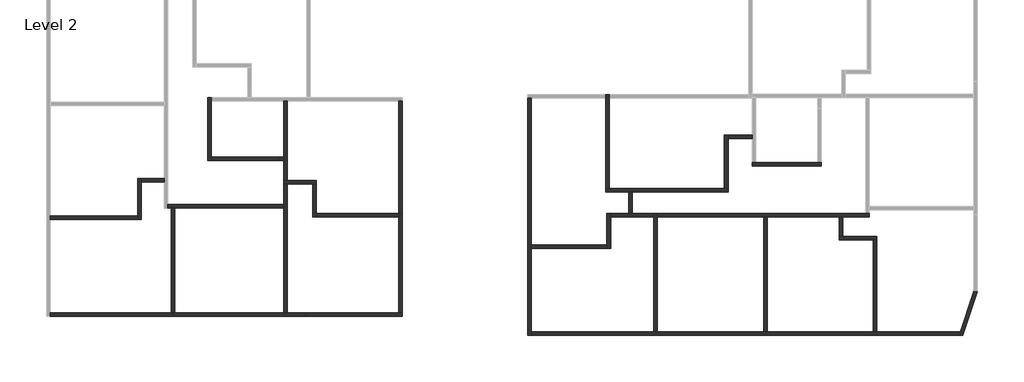
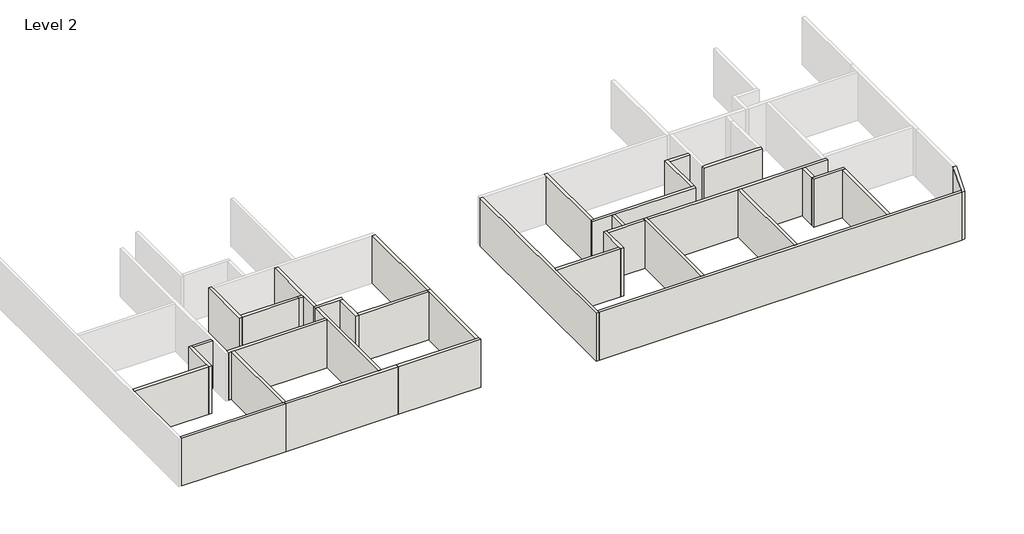
# One storey, part 1 of 2: 36 walls.
"""IFC4 building model written with IfcOpenShell, lengths in millimetres."""

from ifc_helpers import new_model, si_unit, frame, origin, place, context, project, spatial, polyline, outline, extrude, faceted_brep, element, save

model = new_model("IFC4")

# Units and contexts
model_context = context("Model", 3, world=origin())
ifc_project = project(units=[si_unit("LENGTHUNIT", "METRE", prefix="MILLI")], contexts=[model_context])

# Site, building, storey
site = spatial("IfcSite", under=ifc_project)
building = spatial("IfcBuilding", under=site)
storey = spatial("IfcBuildingStorey", under=building, Name="Level 2", Elevation=3000.0)

# Walls
placement = place(None, origin())
element("IfcWall", 1, ObjectType="Generic - 200mm", at=placement, inside=storey, context=model_context, shape_type="Brep", body=[
    faceted_brep([(21449.836337, -2276.2808257, 3000.0), (21249.836337, -2276.2808257, 3000.0), (17730.6041014, -2276.2808257, 3000.0), (17530.6041014, -2276.2808257, 3000.0), (17530.6041014, -2276.2808257, 6360.0), (17730.6041014, -2276.2808257, 6360.0), (21249.836337, -2276.2808257, 6360.0), (21449.836337, -2276.2808257, 6360.0), (21449.836337, -2476.2808257, 3000.0), (21449.836337, -2476.2808257, 6360.0), (17530.6041014, -2476.2808257, 6360.0), (17530.6041014, -2476.2808257, 3000.0)], [[[0, 1, 2, 3, 4, 5, 6, 7]], [[8, 9, 10, 11]], [[3, 2, 1, 0, 8, 11]], [[7, 6, 5, 4, 10, 9]], [[0, 7, 9, 8]], [[4, 3, 11, 10]]]),
])
element("IfcWall", 2, ObjectType="Generic - 200mm", at=placement, inside=storey, context=model_context, shape_type="SweptSolid", body=[
    extrude(outline(polyline([(18379.836337, -5340.0098119), (18379.836337, -11836.6907835), (18179.836337, -11836.6907835), (18179.836337, -5340.0098119), (18379.836337, -5340.0098119)])), frame((0.0, 0.0, 3000.0), z_axis=(0.0, 0.0, 1.0), x_axis=(1.0, 0.0, 0.0)), (0.0, 0.0, 1.0), 3360.0),
])
element("IfcWall", 3, ObjectType="Generic - 200mm", at=placement, inside=storey, context=model_context, shape_type="Brep", body=[
    faceted_brep([(29295.3124022, -11836.6907835, 3000.0), (24588.8612349, -11836.6907835, 3000.0), (24388.8612349, -11836.6907835, 3000.0), (18379.836337, -11836.6907835, 3000.0), (18179.836337, -11836.6907835, 3000.0), (12179.836337, -11836.6907835, 3000.0), (11979.836337, -11836.6907835, 3000.0), (5043.716007, -11836.6907835, 3000.0), (5043.716007, -11836.6907835, 6360.0), (11979.836337, -11836.6907835, 6360.0), (12179.836337, -11836.6907835, 6360.0), (18179.836337, -11836.6907835, 6360.0), (18379.836337, -11836.6907835, 6360.0), (24388.8612349, -11836.6907835, 6360.0), (24588.8612349, -11836.6907835, 6360.0), (29295.3124022, -11836.6907835, 6360.0), (29227.8162902, -12036.6907835, 3000.0), (29227.8162902, -12036.6907835, 6360.0), (5043.716007, -12036.6907835, 6360.0), (5043.716007, -12036.6907835, 3000.0)], [[[0, 1, 2, 3, 4, 5, 6, 7, 8, 9, 10, 11, 12, 13, 14, 15]], [[16, 17, 18, 19]], [[7, 6, 5, 4, 3, 2, 1, 0, 16, 19]], [[15, 14, 13, 12, 11, 10, 9, 8, 18, 17]], [[0, 15, 17, 16]], [[8, 7, 19, 18]]]),
])
element("IfcWall", 4, ObjectType="Generic - 200mm", at=placement, inside=storey, context=model_context, shape_type="Brep", body=[
    faceted_brep([(30069.3799498, -9543.0251929, 3000.0), (29295.3124022, -11836.6907835, 3000.0), (29227.8162902, -12036.6907835, 3000.0), (29227.8162902, -12036.6907835, 6360.0), (29295.3124022, -11836.6907835, 6360.0), (30069.3799498, -9543.0251929, 6360.0), (30269.3799498, -9575.863443, 3000.0), (30269.3799498, -9575.863443, 6360.0), (29438.8985612, -12036.6907835, 6360.0), (29438.8985612, -12036.6907835, 3000.0)], [[[0, 1, 2, 3, 4, 5]], [[6, 7, 8, 9]], [[2, 1, 0, 6, 9]], [[5, 4, 3, 8, 7]], [[0, 5, 7, 6]], [[3, 2, 9, 8]]]),
])
element("IfcWall", 5, ObjectType="Generic - 200mm", at=placement, inside=storey, context=model_context, shape_type="Brep", body=[
    faceted_brep([(24163.3998354, -5140.0098119, 3000.0), (24148.8612349, -5140.0098119, 3000.0), (23948.8612349, -5140.0098119, 3000.0), (12179.836337, -5140.0098119, 3000.0), (12179.836337, -5140.0098119, 6360.0), (23948.8612349, -5140.0098119, 6360.0), (24148.8612349, -5140.0098119, 6360.0), (24163.3998354, -5140.0098119, 6360.0), (24163.3998354, -5340.0098119, 3000.0), (24163.3998354, -5340.0098119, 6360.0), (22668.8612349, -5340.0098119, 6360.0), (22468.8612349, -5340.0098119, 6360.0), (18379.836337, -5340.0098119, 6360.0), (18179.836337, -5340.0098119, 6360.0), (12179.836337, -5340.0098119, 6360.0), (12179.836337, -5340.0098119, 3000.0), (18179.836337, -5340.0098119, 3000.0), (18379.836337, -5340.0098119, 3000.0), (22468.8612349, -5340.0098119, 3000.0), (22668.8612349, -5340.0098119, 3000.0)], [[[0, 1, 2, 3, 4, 5, 6, 7]], [[8, 9, 10, 11, 12, 13, 14, 15, 16, 17, 18, 19]], [[3, 2, 1, 0, 8, 19, 18, 17, 16, 15]], [[7, 6, 5, 4, 14, 13, 12, 11, 10, 9]], [[0, 7, 9, 8]], [[4, 3, 15, 14]]]),
])
element("IfcWall", 6, ObjectType="Generic - 200mm", at=placement, inside=storey, context=model_context, shape_type="Brep", body=[
    faceted_brep([(4843.716007, 1379.9901881, 3000.0), (4843.716007, -12036.6907835, 3000.0), (4843.716007, -12036.6907835, 6360.0), (4843.716007, 1379.9901881, 6360.0), (5043.716007, 1379.9901881, 3000.0), (5043.716007, 1379.9901881, 6360.0), (5043.716007, -6920.0098119, 6360.0), (5043.716007, -7120.0098119, 6360.0), (5043.716007, -11836.6907835, 6360.0), (5043.716007, -12036.6907835, 6360.0), (5043.716007, -12036.6907835, 3000.0), (5043.716007, -11836.6907835, 3000.0), (5043.716007, -7120.0098119, 3000.0), (5043.716007, -6920.0098119, 3000.0)], [[[0, 1, 2, 3]], [[4, 5, 6, 7, 8, 9, 10, 11, 12, 13]], [[1, 0, 4, 13, 12, 11, 10]], [[3, 2, 9, 8, 7, 6, 5]], [[2, 1, 10, 9]], [[0, 3, 5, 4]]]),
])
element("IfcWall", 7, ObjectType="Generic - 200mm", at=placement, inside=storey, context=model_context, shape_type="Brep", body=[
    faceted_brep([(9268.8612349, -3940.0098119, 3000.0), (10568.8612349, -3940.0098119, 3000.0), (10768.8612349, -3940.0098119, 3000.0), (16170.6041014, -3940.0098119, 3000.0), (16170.6041014, -3940.0098119, 6360.0), (10768.8612349, -3940.0098119, 6360.0), (10568.8612349, -3940.0098119, 6360.0), (9268.8612349, -3940.0098119, 6360.0), (9268.8612349, -3740.0098119, 3000.0), (9268.8612349, -3740.0098119, 6360.0), (9468.8612349, -3740.0098119, 6360.0), (15970.6041014, -3740.0098119, 6360.0), (16170.6041014, -3740.0098119, 6360.0), (16170.6041014, -3740.0098119, 3000.0), (15970.6041014, -3740.0098119, 3000.0), (9468.8612349, -3740.0098119, 3000.0), (16170.6041014, -3894.2728831, 3000.0)], [[[0, 1, 2, 3, 4, 5, 6, 7]], [[8, 9, 10, 11, 12, 13, 14, 15]], [[3, 2, 1, 0, 8, 15, 14, 13, 16]], [[7, 6, 5, 4, 12, 11, 10, 9]], [[4, 3, 16, 13, 12]], [[0, 7, 9, 8]]]),
])
element("IfcWall", 8, ObjectType="Generic - 200mm", at=placement, inside=storey, context=model_context, shape_type="Brep", body=[
    faceted_brep([(16170.6041014, -3740.0098119, 3000.0), (16170.6041014, -3694.2728831, 3000.0), (16170.6041014, -920.524372, 3000.0), (16170.6041014, -720.524372, 3000.0), (16170.6041014, -720.524372, 6360.0), (16170.6041014, -920.524372, 6360.0), (16170.6041014, -3740.0098119, 6360.0), (15970.6041014, -3740.0098119, 3000.0), (15970.6041014, -3740.0098119, 6360.0), (15970.6041014, -720.524372, 6360.0), (15970.6041014, -720.524372, 3000.0)], [[[0, 1, 2, 3, 4, 5, 6]], [[7, 8, 9, 10]], [[3, 2, 1, 0, 7, 10]], [[6, 5, 4, 9, 8]], [[0, 6, 8, 7]], [[4, 3, 10, 9]]]),
])
element("IfcWall", 9, ObjectType="Generic - 200mm", at=placement, inside=storey, context=model_context, shape_type="SweptSolid", body=[
    extrude(outline(polyline([(17530.6041014, -920.524372), (16170.6041014, -920.524372), (16170.6041014, -720.524372), (17530.6041014, -720.524372), (17530.6041014, -920.524372)])), frame((0.0, 0.0, 3000.0), z_axis=(0.0, 0.0, 1.0), x_axis=(1.0, 0.0, 0.0)), (0.0, 0.0, 1.0), 3360.0),
])
element("IfcWall", 10, ObjectType="Generic - 200mm", at=placement, inside=storey, context=model_context, shape_type="Brep", body=[
    faceted_brep([(22468.8612349, -6641.2808257, 3000.0), (24388.8612349, -6641.2808257, 3000.0), (24588.8612349, -6641.2808257, 3000.0), (24588.8612349, -6641.2808257, 6360.0), (24388.8612349, -6641.2808257, 6360.0), (22468.8612349, -6641.2808257, 6360.0), (22468.8612349, -6441.2808257, 3000.0), (22468.8612349, -6441.2808257, 6360.0), (22668.8612349, -6441.2808257, 6360.0), (24588.8612349, -6441.2808257, 6360.0), (24588.8612349, -6441.2808257, 3000.0), (22668.8612349, -6441.2808257, 3000.0)], [[[0, 1, 2, 3, 4, 5]], [[6, 7, 8, 9, 10, 11]], [[2, 1, 0, 6, 11, 10]], [[5, 4, 3, 9, 8, 7]], [[3, 2, 10, 9]], [[0, 5, 7, 6]]]),
])
element("IfcWall", 11, ObjectType="Generic - 200mm", at=placement, inside=storey, context=model_context, shape_type="SweptSolid", body=[
    extrude(outline(polyline([(24388.8612349, -11836.6907835), (24388.8612349, -6641.2808257), (24588.8612349, -6641.2808257), (24588.8612349, -11836.6907835), (24388.8612349, -11836.6907835)])), frame((0.0, 0.0, 3000.0), z_axis=(0.0, 0.0, 1.0), x_axis=(1.0, 0.0, 0.0)), (0.0, 0.0, 1.0), 3360.0),
])
element("IfcWall", 12, ObjectType="Generic - 200mm", at=placement, inside=storey, context=model_context, shape_type="SweptSolid", body=[
    extrude(outline(polyline([(22668.8612349, -5340.0098119), (22668.8612349, -6441.2808257), (22468.8612349, -6441.2808257), (22468.8612349, -5340.0098119), (22668.8612349, -5340.0098119)])), frame((0.0, 0.0, 3000.0), z_axis=(0.0, 0.0, 1.0), x_axis=(1.0, 0.0, 0.0)), (0.0, 0.0, 1.0), 3360.0),
])
element("IfcWall", 13, ObjectType="Generic - 200mm", at=placement, inside=storey, context=model_context, shape_type="Brep", body=[
    faceted_brep([(9268.8612349, 1579.9901881, 3000.0), (9268.8612349, 1379.9901881, 3000.0), (9268.8612349, -3740.0098119, 3000.0), (9268.8612349, -3740.0098119, 6360.0), (9268.8612349, 1379.9901881, 6360.0), (9268.8612349, 1579.9901881, 6360.0), (9468.8612349, 1579.9901881, 3000.0), (9468.8612349, 1579.9901881, 6360.0), (9468.8612349, 1579.475628, 6360.0), (9468.8612349, 1379.475628, 6360.0), (9468.8612349, -3740.0098119, 6360.0), (9468.8612349, -3740.0098119, 3000.0), (9468.8612349, 1379.475628, 3000.0), (9468.8612349, 1579.475628, 3000.0)], [[[0, 1, 2, 3, 4, 5]], [[6, 7, 8, 9, 10, 11, 12, 13]], [[2, 1, 0, 6, 13, 12, 11]], [[5, 4, 3, 10, 9, 8, 7]], [[3, 2, 11, 10]], [[0, 5, 7, 6]]]),
])
element("IfcWall", 14, ObjectType="Generic - 200mm", at=placement, inside=storey, context=model_context, shape_type="SweptSolid", body=[
    extrude(outline(polyline([(5043.716007, -6920.0098119), (9328.8612349, -6920.0098119), (9328.8612349, -7120.0098119), (5043.716007, -7120.0098119), (5043.716007, -6920.0098119)])), frame((0.0, 0.0, 3000.0), z_axis=(0.0, 0.0, 1.0), x_axis=(1.0, 0.0, 0.0)), (0.0, 0.0, 1.0), 3360.0),
])
element("IfcWall", 15, ObjectType="Generic - 200mm", at=placement, inside=storey, context=model_context, shape_type="Brep", body=[
    faceted_brep([(-2430.3449834, -5140.1378151, 3000.0), (-2430.3449834, -5340.1378151, 3000.0), (-2430.3449834, -10758.643998, 3000.0), (-2430.3449834, -10758.643998, 6360.0), (-2430.3449834, -5340.1378151, 6360.0), (-2430.3449834, -5140.1378151, 6360.0), (-2230.3449834, -5140.1378151, 3000.0), (-2230.3449834, -5140.1378151, 6360.0), (-2230.3449834, -10758.643998, 6360.0), (-2230.3449834, -10758.643998, 3000.0)], [[[0, 1, 2, 3, 4, 5]], [[6, 7, 8, 9]], [[2, 1, 0, 6, 9]], [[5, 4, 3, 8, 7]], [[3, 2, 9, 8]], [[0, 5, 7, 6]]]),
])
element("IfcWall", 16, ObjectType="Generic - 200mm", at=placement, inside=storey, context=model_context, shape_type="Brep", body=[
    faceted_brep([(-2230.3449834, -10758.643998, 3000.0), (-2430.3449834, -10758.643998, 3000.0), (-7730.3449834, -10758.643998, 3000.0), (-7730.3449834, -10758.643998, 6360.0), (-2430.3449834, -10758.643998, 6360.0), (-2230.3449834, -10758.643998, 6360.0), (-2230.3449834, -10958.643998, 3000.0), (-2230.3449834, -10958.643998, 6360.0), (-7730.3449834, -10958.643998, 6360.0), (-7730.3449834, -10958.643998, 3000.0), (-7730.3449834, -10932.392509, 3000.0), (-7730.3449834, -10759.1627129, 3000.0), (-7730.3449834, -10759.1627129, 6360.0)], [[[0, 1, 2, 3, 4, 5]], [[6, 7, 8, 9]], [[2, 1, 0, 6, 9, 10, 11]], [[3, 2, 11, 10, 9, 8, 12]], [[5, 4, 3, 12, 8, 7]], [[0, 5, 7, 6]]]),
])
element("IfcWall", 17, ObjectType="Generic - 200mm", at=placement, inside=storey, context=model_context, shape_type="Brep", body=[
    faceted_brep([(-7730.3449834, -10759.1627129, 3000.0), (-8730.3449834, -10759.1627129, 3000.0), (-8930.3449834, -10759.1627129, 3000.0), (-15109.8304233, -10759.1627129, 3000.0), (-15209.8304233, -10759.1627129, 3000.0), (-15209.8304233, -10759.1627129, 6360.0), (-15109.8304233, -10759.1627129, 6360.0), (-8930.3449834, -10759.1627129, 6360.0), (-8730.3449834, -10759.1627129, 6360.0), (-7730.3449834, -10759.1627129, 6360.0), (-7730.3449834, -10959.1627129, 3000.0), (-7730.3449834, -10959.1627129, 6360.0), (-15209.8304233, -10959.1627129, 6360.0), (-15209.8304233, -10959.1627129, 3000.0), (-7730.3449834, -10932.911224, 3000.0), (-7730.3449834, -10958.643998, 3000.0), (-15209.8304233, -10932.911224, 3000.0), (-15209.8304233, -10759.6814279, 3000.0), (-15209.8304233, -10759.6814279, 6360.0), (-7730.3449834, -10958.643998, 6360.0)], [[[0, 1, 2, 3, 4, 5, 6, 7, 8, 9]], [[10, 11, 12, 13]], [[4, 3, 2, 1, 0, 14, 15, 10, 13, 16, 17]], [[5, 4, 17, 16, 13, 12, 18]], [[9, 8, 7, 6, 5, 18, 12, 11, 19]], [[0, 9, 19, 11, 10, 15, 14]]]),
])
element("IfcWall", 18, ObjectType="Generic - 200mm", at=placement, inside=storey, context=model_context, shape_type="Brep", body=[
    faceted_brep([(-15209.8304233, -10759.6814279, 3000.0), (-15309.8304233, -10759.6814279, 3000.0), (-22146.5113948, -10759.6814279, 3000.0), (-22146.5113948, -10759.6814279, 6360.0), (-15309.8304233, -10759.6814279, 6360.0), (-15209.8304233, -10759.6814279, 6360.0), (-15209.8304233, -10959.6814279, 3000.0), (-15209.8304233, -10959.6814279, 6360.0), (-22146.5113948, -10959.6814279, 6360.0), (-22146.5113948, -10959.6814279, 3000.0), (-15209.8304233, -10933.429939, 3000.0), (-15209.8304233, -10959.1627129, 3000.0), (-15209.8304233, -10959.1627129, 6360.0)], [[[0, 1, 2, 3, 4, 5]], [[6, 7, 8, 9]], [[2, 1, 0, 10, 11, 6, 9]], [[5, 4, 3, 8, 7, 12]], [[0, 5, 12, 7, 6, 11, 10]], [[3, 2, 9, 8]]]),
])
element("IfcWall", 19, ObjectType="Generic - 200mm", at=placement, inside=storey, context=model_context, shape_type="Brep", body=[
    faceted_brep([(-13026.101437, -2140.1378151, 3000.0), (-13026.101437, -1940.1378151, 3000.0), (-13026.101437, 1200.8372871, 3000.0), (-13026.101437, 1400.8372871, 3000.0), (-13026.101437, 1400.8372871, 6360.0), (-13026.101437, 1200.8372871, 6360.0), (-13026.101437, -1940.1378151, 6360.0), (-13026.101437, -2140.1378151, 6360.0), (-13226.101437, -2140.1378151, 3000.0), (-13226.101437, -2140.1378151, 6360.0), (-13226.101437, 1400.8372871, 6360.0), (-13226.101437, 1400.8372871, 3000.0)], [[[0, 1, 2, 3, 4, 5, 6, 7]], [[8, 9, 10, 11]], [[3, 2, 1, 0, 8, 11]], [[7, 6, 5, 4, 10, 9]], [[0, 7, 9, 8]], [[4, 3, 11, 10]]]),
])
element("IfcWall", 20, ObjectType="Generic - 200mm", at=placement, inside=storey, context=model_context, shape_type="Brep", body=[
    faceted_brep([(-15489.8304233, -4839.1627129, 3000.0), (-15309.8304233, -4839.1627129, 3000.0), (-15109.8304233, -4839.1627129, 3000.0), (-8930.3449834, -4839.1627129, 3000.0), (-8930.3449834, -4839.1627129, 6360.0), (-15109.8304233, -4839.1627129, 6360.0), (-15309.8304233, -4839.1627129, 6360.0), (-15489.8304233, -4839.1627129, 6360.0), (-15489.8304233, -4639.1627129, 3000.0), (-15489.8304233, -4639.1627129, 6360.0), (-8930.3449834, -4639.1627129, 6360.0), (-8930.3449834, -4639.1627129, 3000.0)], [[[0, 1, 2, 3, 4, 5, 6, 7]], [[8, 9, 10, 11]], [[3, 2, 1, 0, 8, 11]], [[7, 6, 5, 4, 10, 9]], [[4, 3, 11, 10]], [[0, 7, 9, 8]]]),
])
element("IfcWall", 21, ObjectType="Generic - 200mm", at=placement, inside=storey, context=model_context, shape_type="SweptSolid", body=[
    extrude(outline(polyline([(-13026.101437, -1940.1378151), (-9250.3449834, -1940.1378151), (-9250.3449834, -2140.1378151), (-13026.101437, -2140.1378151), (-13026.101437, -1940.1378151)])), frame((0.0, 0.0, 3000.0), z_axis=(0.0, 0.0, 1.0), x_axis=(1.0, 0.0, 0.0)), (0.0, 0.0, 1.0), 3360.0),
])
element("IfcWall", 22, ObjectType="Generic - 200mm", at=placement, inside=storey, context=model_context, shape_type="SweptSolid", body=[
    extrude(outline(polyline([(-8930.3449834, -2140.1378151), (-9250.3449834, -2140.1378151), (-9250.3449834, -1940.1378151), (-8930.3449834, -1940.1378151), (-8930.3449834, -2140.1378151)])), frame((0.0, 0.0, 3000.0), z_axis=(0.0, 0.0, 1.0), x_axis=(1.0, 0.0, 0.0)), (0.0, 0.0, 1.0), 3360.0),
])
element("IfcWall", 23, ObjectType="Generic - 200mm", at=placement, inside=storey, context=model_context, shape_type="SweptSolid", body=[
    extrude(outline(polyline([(-2430.3449834, -5140.1378151), (-2430.3449834, 1200.8372871), (-2230.3449834, 1200.8372871), (-2230.3449834, -5140.1378151), (-2430.3449834, -5140.1378151)])), frame((0.0, 0.0, 3000.0), z_axis=(0.0, 0.0, 1.0), x_axis=(1.0, 0.0, 0.0)), (0.0, 0.0, 1.0), 3360.0),
])
element("IfcWall", 24, ObjectType="Generic - 200mm", at=placement, inside=storey, context=model_context, shape_type="Brep", body=[
    faceted_brep([(-8930.3449834, -3480.1378151, 3000.0), (-8730.3449834, -3480.1378151, 3000.0), (-7295.3449834, -3480.1378151, 3000.0), (-7095.3449834, -3480.1378151, 3000.0), (-7095.3449834, -3480.1378151, 6360.0), (-7295.3449834, -3480.1378151, 6360.0), (-8730.3449834, -3480.1378151, 6360.0), (-8930.3449834, -3480.1378151, 6360.0), (-8930.3449834, -3280.1378151, 3000.0), (-8930.3449834, -3280.1378151, 6360.0), (-8730.3449834, -3280.1378151, 6360.0), (-7095.3449834, -3280.1378151, 6360.0), (-7095.3449834, -3280.1378151, 3000.0), (-8730.3449834, -3280.1378151, 3000.0), (-8930.3449834, -3453.8863261, 3000.0)], [[[0, 1, 2, 3, 4, 5, 6, 7]], [[8, 9, 10, 11, 12, 13]], [[3, 2, 1, 0, 14, 8, 13, 12]], [[7, 6, 5, 4, 11, 10, 9]], [[0, 7, 9, 8, 14]], [[4, 3, 12, 11]]]),
])
element("IfcWall", 25, ObjectType="Generic - 200mm", at=placement, inside=storey, context=model_context, shape_type="Brep", body=[
    faceted_brep([(-8930.3449834, -3480.1378151, 3000.0), (-8930.3449834, -4639.1627129, 3000.0), (-8930.3449834, -4839.1627129, 3000.0), (-8930.3449834, -10759.1627129, 3000.0), (-8930.3449834, -10759.1627129, 6360.0), (-8930.3449834, -4839.1627129, 6360.0), (-8930.3449834, -4639.1627129, 6360.0), (-8930.3449834, -3480.1378151, 6360.0), (-8730.3449834, -3480.1378151, 3000.0), (-8730.3449834, -3480.1378151, 6360.0), (-8730.3449834, -10759.1627129, 6360.0), (-8730.3449834, -10759.1627129, 3000.0)], [[[0, 1, 2, 3, 4, 5, 6, 7]], [[8, 9, 10, 11]], [[3, 2, 1, 0, 8, 11]], [[7, 6, 5, 4, 10, 9]], [[4, 3, 11, 10]], [[0, 7, 9, 8]]]),
])
element("IfcWall", 26, ObjectType="Generic - 200mm", at=placement, inside=storey, context=model_context, shape_type="Brep", body=[
    faceted_brep([(-8730.3449834, -3280.1378151, 3000.0), (-8730.3449834, 1200.8372871, 3000.0), (-8730.3449834, 1200.8372871, 6360.0), (-8730.3449834, -3280.1378151, 6360.0), (-8930.3449834, -3280.1378151, 3000.0), (-8930.3449834, -3280.1378151, 6360.0), (-8930.3449834, -2140.1378151, 6360.0), (-8930.3449834, -1940.1378151, 6360.0), (-8930.3449834, 1200.8372871, 6360.0), (-8930.3449834, 1200.8372871, 3000.0), (-8930.3449834, -1940.1378151, 3000.0), (-8930.3449834, -2140.1378151, 3000.0), (-8930.3449834, -3253.8863261, 3000.0)], [[[0, 1, 2, 3]], [[4, 5, 6, 7, 8, 9, 10, 11, 12]], [[1, 0, 4, 12, 11, 10, 9]], [[3, 2, 8, 7, 6, 5]], [[0, 3, 5, 4]], [[2, 1, 9, 8]]]),
])
element("IfcWall", 27, ObjectType="Generic - 200mm", at=placement, inside=storey, context=model_context, shape_type="Brep", body=[
    faceted_brep([(-7295.3449834, -3480.1378151, 3000.0), (-7295.3449834, -5340.1378151, 3000.0), (-7295.3449834, -5340.1378151, 6360.0), (-7295.3449834, -3480.1378151, 6360.0), (-7095.3449834, -3480.1378151, 3000.0), (-7095.3449834, -3480.1378151, 6360.0), (-7095.3449834, -5140.1378151, 6360.0), (-7095.3449834, -5340.1378151, 6360.0), (-7095.3449834, -5340.1378151, 3000.0), (-7095.3449834, -5140.1378151, 3000.0)], [[[0, 1, 2, 3]], [[4, 5, 6, 7, 8, 9]], [[1, 0, 4, 9, 8]], [[3, 2, 7, 6, 5]], [[2, 1, 8, 7]], [[0, 3, 5, 4]]]),
])
element("IfcWall", 28, ObjectType="Generic - 200mm", at=placement, inside=storey, context=model_context, shape_type="SweptSolid", body=[
    extrude(outline(polyline([(-2430.3449834, -5340.1378151), (-7095.3449834, -5340.1378151), (-7095.3449834, -5140.1378151), (-2430.3449834, -5140.1378151), (-2430.3449834, -5340.1378151)])), frame((0.0, 0.0, 3000.0), z_axis=(0.0, 0.0, 1.0), x_axis=(1.0, 0.0, 0.0)), (0.0, 0.0, 1.0), 3360.0),
])
element("IfcWall", 29, ObjectType="Generic - 200mm", at=placement, inside=storey, context=model_context, shape_type="Brep", body=[
    faceted_brep([(-17191.101437, -3159.1627129, 3000.0), (-17191.101437, -5279.1627129, 3000.0), (-17191.101437, -5479.1627129, 3000.0), (-17191.101437, -5479.1627129, 6360.0), (-17191.101437, -5279.1627129, 6360.0), (-17191.101437, -3159.1627129, 6360.0), (-16991.101437, -3159.1627129, 3000.0), (-16991.101437, -3159.1627129, 6360.0), (-16991.101437, -3359.1627129, 6360.0), (-16991.101437, -5479.1627129, 6360.0), (-16991.101437, -5479.1627129, 3000.0), (-16991.101437, -3359.1627129, 3000.0)], [[[0, 1, 2, 3, 4, 5]], [[6, 7, 8, 9, 10, 11]], [[2, 1, 0, 6, 11, 10]], [[5, 4, 3, 9, 8, 7]], [[3, 2, 10, 9]], [[0, 5, 7, 6]]]),
])
element("IfcWall", 30, ObjectType="Generic - 200mm", at=placement, inside=storey, context=model_context, shape_type="SweptSolid", body=[
    extrude(outline(polyline([(-22146.5113948, -5279.1627129), (-17191.101437, -5279.1627129), (-17191.101437, -5479.1627129), (-22146.5113948, -5479.1627129), (-22146.5113948, -5279.1627129)])), frame((0.0, 0.0, 3000.0), z_axis=(0.0, 0.0, 1.0), x_axis=(1.0, 0.0, 0.0)), (0.0, 0.0, 1.0), 3360.0),
])
element("IfcWall", 31, ObjectType="Generic - 200mm", at=placement, inside=storey, context=model_context, shape_type="SweptSolid", body=[
    extrude(outline(polyline([(-15689.8304233, -3359.1627129), (-16991.101437, -3359.1627129), (-16991.101437, -3159.1627129), (-15689.8304233, -3159.1627129), (-15689.8304233, -3359.1627129)])), frame((0.0, 0.0, 3000.0), z_axis=(0.0, 0.0, 1.0), x_axis=(1.0, 0.0, 0.0)), (0.0, 0.0, 1.0), 3360.0),
])
element("IfcWall", 32, ObjectType="Generic - 200mm", at=placement, inside=storey, context=model_context, shape_type="SweptSolid", body=[
    extrude(outline(polyline([(-15309.8304233, -10759.6814279), (-15309.8304233, -4839.1627129), (-15109.8304233, -4839.1627129), (-15109.8304233, -10759.1627129), (-15209.8304233, -10759.1627129), (-15209.8304233, -10759.6814279), (-15309.8304233, -10759.6814279)])), frame((0.0, 0.0, 3000.0), z_axis=(0.0, 0.0, 1.0), x_axis=(1.0, 0.0, 0.0)), (0.0, 0.0, 1.0), 3360.0),
])
element("IfcWall", 33, ObjectType="Generic - 200mm", at=placement, inside=storey, context=model_context, shape_type="Brep", body=[
    faceted_brep([(11979.836337, -5136.6907835, 3000.0), (11979.836337, -5336.6907835, 3000.0), (11979.836337, -11836.6907835, 3000.0), (11979.836337, -11836.6907835, 6360.0), (11979.836337, -5336.6907835, 6360.0), (11979.836337, -5136.6907835, 6360.0), (12179.836337, -5136.6907835, 3000.0), (12179.836337, -5136.6907835, 6360.0), (12179.836337, -5140.0098119, 6360.0), (12179.836337, -5340.0098119, 6360.0), (12179.836337, -11836.6907835, 6360.0), (12179.836337, -11836.6907835, 3000.0), (12179.836337, -5340.0098119, 3000.0), (12179.836337, -5140.0098119, 3000.0)], [[[0, 1, 2, 3, 4, 5]], [[6, 7, 8, 9, 10, 11, 12, 13]], [[2, 1, 0, 6, 13, 12, 11]], [[5, 4, 3, 10, 9, 8, 7]], [[3, 2, 11, 10]], [[0, 5, 7, 6]]]),
])
element("IfcWall", 34, ObjectType="Generic - 200mm", at=placement, inside=storey, context=model_context, shape_type="Brep", body=[
    faceted_brep([(9528.8612349, -7120.0098119, 3000.0), (9528.8612349, -5336.6907835, 3000.0), (9528.8612349, -5136.6907835, 3000.0), (9528.8612349, -5136.6907835, 6360.0), (9528.8612349, -5336.6907835, 6360.0), (9528.8612349, -7120.0098119, 6360.0), (9328.8612349, -7120.0098119, 3000.0), (9328.8612349, -7120.0098119, 6360.0), (9328.8612349, -6920.0098119, 6360.0), (9328.8612349, -5136.6907835, 6360.0), (9328.8612349, -5136.6907835, 3000.0), (9328.8612349, -6920.0098119, 3000.0)], [[[0, 1, 2, 3, 4, 5]], [[6, 7, 8, 9, 10, 11]], [[2, 1, 0, 6, 11, 10]], [[5, 4, 3, 9, 8, 7]], [[3, 2, 10, 9]], [[0, 5, 7, 6]]]),
])
element("IfcWall", 35, ObjectType="Generic - 200mm", at=placement, inside=storey, context=model_context, shape_type="Brep", body=[
    faceted_brep([(9528.8612349, -5336.6907835, 3000.0), (11979.836337, -5336.6907835, 3000.0), (11979.836337, -5336.6907835, 6360.0), (9528.8612349, -5336.6907835, 6360.0), (9528.8612349, -5136.6907835, 3000.0), (9528.8612349, -5136.6907835, 6360.0), (10568.8612349, -5136.6907835, 6360.0), (10768.8612349, -5136.6907835, 6360.0), (11979.836337, -5136.6907835, 6360.0), (11979.836337, -5136.6907835, 3000.0), (10768.8612349, -5136.6907835, 3000.0), (10568.8612349, -5136.6907835, 3000.0)], [[[0, 1, 2, 3]], [[4, 5, 6, 7, 8, 9, 10, 11]], [[1, 0, 4, 11, 10, 9]], [[3, 2, 8, 7, 6, 5]], [[0, 3, 5, 4]], [[2, 1, 9, 8]]]),
])
element("IfcWall", 36, ObjectType="Generic - 200mm", at=placement, inside=storey, context=model_context, shape_type="SweptSolid", body=[
    extrude(outline(polyline([(10568.8612349, -5136.6907835), (10568.8612349, -3940.0098119), (10768.8612349, -3940.0098119), (10768.8612349, -5136.6907835), (10568.8612349, -5136.6907835)])), frame((0.0, 0.0, 3000.0), z_axis=(0.0, 0.0, 1.0), x_axis=(1.0, 0.0, 0.0)), (0.0, 0.0, 1.0), 3360.0),
])

save(model, "model.ifc")

# Revit data of these elements
# Type "Generic - 200mm"
#   Layers, outside or top first: 20 cm no material (function 1)
# Elements 1, 2, 3, 4, 5, 6, 7, 8, 9, 10, 11, 12, 13, 14, 15, 16, 17, 18, 19, 20, 21, 22, 23, 24, 25, 26, 27, 28, 29, 30, 31, 32, 33, 34, 35, 36 (IfcWall, "Generic - 200mm")
#   Top Offset = 0 cm
#   Base Offset = 0 cm
#   wall height = 336 cm
#   Phase Created = New Construction
#   Base Constraint = Level 2
#   Top Constraint = Level 3
#   Materials on its faces: "Default Wall"
# Materials
#   "Default Wall": class "Miscellaneous", colour RGB 128 128 128, transparency 0, Cost = 0
# Room, not placed, phase "New Construction", upper offset 0 cm, lower offset 0 cm
#   Number = "140"
#   Name = "2"
# Room, not placed, phase "New Construction", upper offset 0 cm, lower offset 0 cm
#   Number = "141"
#   Name = "3"
# Room at (-10319.93, 6237.76) mm, phase "New Construction", upper level "Level 2", upper offset 243.84 cm, lower offset 0 cm
#   Number = "142"
#   Name = "Room"
# Room at (-20464.33, 11799.355) mm, phase "New Construction", upper level "Level 2", upper offset 243.84 cm, lower offset 0 cm
#   Number = "143"
#   Name = "Room"
# Room at (-5737.571, -7303.63) mm, phase "New Construction", upper level "Level 2", upper offset 243.84 cm, lower offset 0 cm
#   Number = "144"
#   Name = "Room"
# Room at (-5098.071, -1353.454) mm, phase "New Construction", upper level "Level 2", upper offset 243.84 cm, lower offset 0 cm
#   Number = "145"
#   Name = "Room"
# Area at (-11657.115, 14542.776) mm, upper offset 243.84 cm, lower offset 0 cm
#   Number = "10"
#   Name = "Area"
# Room at (-19577.139, -1804.795) mm, phase "New Construction", upper level "Level 2", upper offset 243.84 cm, lower offset 0 cm
#   Number = "146"
#   Name = "Room"
# Room at (-18721.372, 5082.955) mm, phase "New Construction", upper level "Level 2", upper offset 243.84 cm, lower offset 0 cm
#   Number = "147"
#   Name = "Room"
# Room at (-13880.202, 12312.878) mm, phase "New Construction", upper level "Level 2", upper offset 243.84 cm, lower offset 0 cm
#   Number = "148"
#   Name = "Room"
# Room at (20668.363, 5082.955) mm, phase "New Construction", upper level "Level 2", upper offset 243.84 cm, lower offset 0 cm
#   Number = "149"
#   Name = "9"
# Room at (27272.961, 5082.955) mm, phase "New Construction", upper level "Level 2", upper offset 243.84 cm, lower offset 0 cm
#   Number = "150"
#   Name = "1"
# Room at (27272.961, -1353.454) mm, phase "New Construction", upper level "Level 2", upper offset 243.84 cm, lower offset 0 cm
#   Number = "151"
#   Name = "2"
# Room at (27272.961, -8176.995) mm, phase "New Construction", upper level "Level 2", upper offset 243.84 cm, lower offset 0 cm
#   Number = "152"
#   Name = "3"
# Room at (21743.53, -9098.567) mm, phase "New Construction", upper level "Level 2", upper offset 243.84 cm, lower offset 0 cm
#   Number = "153"
#   Name = "4"
# Room at (14985.336, -8176.995) mm, phase "New Construction", upper level "Level 2", upper offset 243.84 cm, lower offset 0 cm
#   Number = "154"
#   Name = "5"
# Room at (8687.927, -8976.995) mm, phase "New Construction", upper level "Level 2", upper offset 243.84 cm, lower offset 0 cm
#   Number = "155"
#   Name = "6"
# Room at (13142.192, -1353.454) mm, phase "New Construction", upper level "Level 2", upper offset 243.84 cm, lower offset 0 cm
#   Number = "156"
#   Name = "8"
# Room at (7305.569, -1804.795) mm, phase "New Construction", upper level "Level 2", upper offset 243.84 cm, lower offset 0 cm
#   Number = "157"
#   Name = "7"
# Room at (-12277.834, -7303.63) mm, phase "New Construction", upper level "Level 2", upper offset 243.84 cm, lower offset 0 cm
#   Number = "158"
#   Name = "Room"
# Room at (-18721.372, -7303.63) mm, phase "New Construction", upper level "Level 2", upper offset 243.84 cm, lower offset 0 cm
#   Number = "159"
#   Name = "Room"
